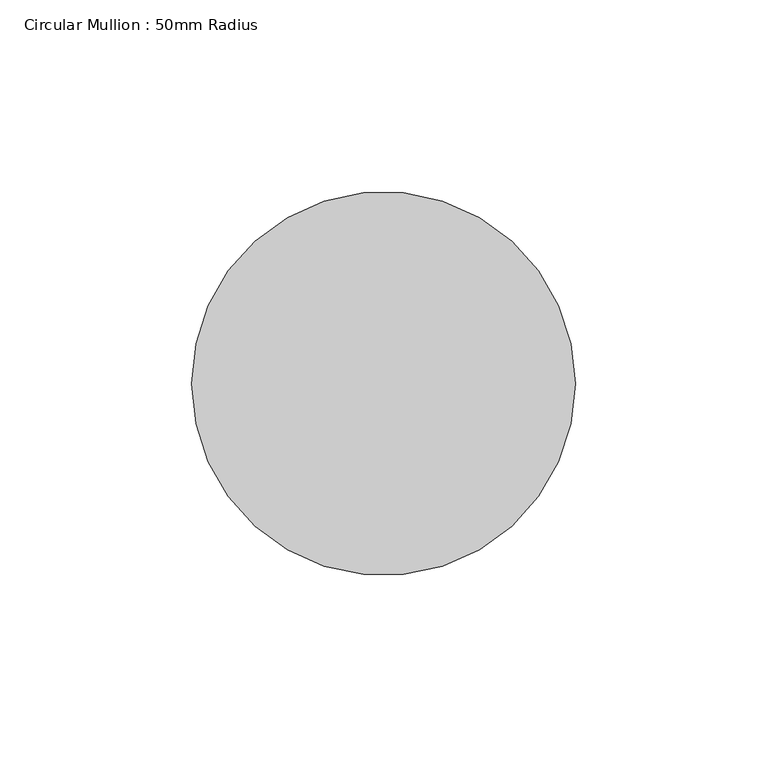
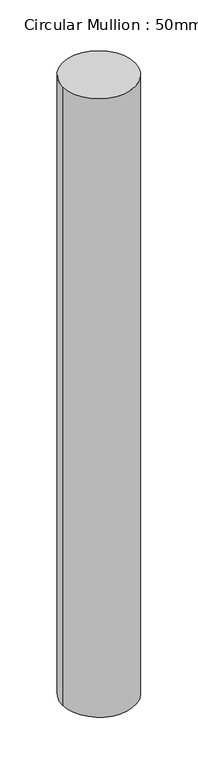
"""IFC4 building model written with IfcOpenShell, lengths in millimetres: member geometry, Circular Mullion : 50mm Radius."""

from ifc_helpers import new_model, si_unit, point, frame, origin, origin_2d, place, context, project, spatial, circle_curve, trimmed, segment, composite_curve, outline, extrude, source, transform, mapped, element, save


def circular_mullion_50mm_radius_92986f1a(model_context):
    return source(origin(), model_context, "Body", "SweptSolid", [
        extrude(outline(composite_curve([segment(trimmed(circle_curve(origin_2d(), 50.0), [point((50.0, 0.0))], [point((-50.0, 0.0))], False, "CARTESIAN"), True, "CONTINUOUS"), segment(trimmed(circle_curve(origin_2d(), 50.0), [point((-50.0, 0.0))], [point((50.0, 0.0))], False, "CARTESIAN"), True, "CONTINUOUS")], self_intersect=False)), frame((0.0, 0.0, -901.3412912), z_axis=(0.0, 0.0, 1.0), x_axis=(1.0, 0.0, 0.0)), (0.0, 0.0, 1.0), 901.3412912),
    ])


if __name__ == "__main__":
    model = new_model("IFC4")
    model_context = context("Model", 3, world=origin())
    ifc_project = project(units=[si_unit("LENGTHUNIT", "METRE", prefix="MILLI")], contexts=[model_context])
    site = spatial("IfcSite", under=ifc_project)
    building = spatial("IfcBuilding", under=site)
    placement = place(None, origin())
    circular_mullion_50mm_radius_shape = circular_mullion_50mm_radius_92986f1a(model_context)
    element("IfcMember", 1, ObjectType="Circular Mullion : 50mm Radius", at=placement, inside=building, context=model_context, shape_type="MappedRepresentation", body=[
        mapped(circular_mullion_50mm_radius_shape, transform((0.0, 0.0, 0.0), x_axis=(1.0, 0.0, 0.0), y_axis=(0.0, 1.0, 0.0), z_axis=(0.0, 0.0, 1.0))),
    ])
    save(model, "model.ifc")

# Revit data of these elements
# Type "Circular Mullion : 50mm Radius"
#   built-in parameter 1007350 = 0.164042 (stored number, unit not read)
# Element 1 (IfcMember, "Circular Mullion : 50mm Radius")
#   Materials on its faces: "Aluminium"
# Materials
#   "Aluminium": class "Metal", colour RGB 247 247 247, transparency 0, Description = "Aluminium 6061", Cost = 0
